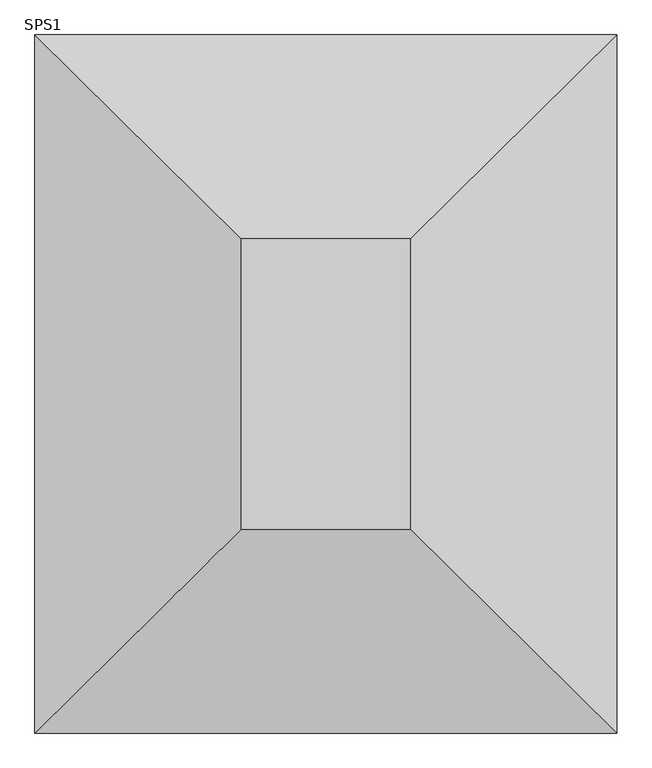
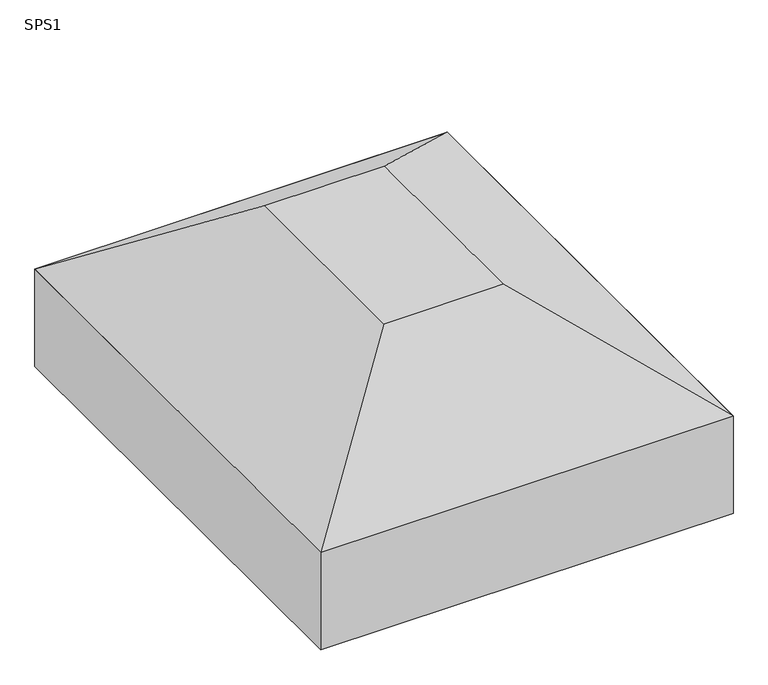
"""IFC4 building model written with IfcOpenShell, lengths in millimetres: fastener geometry, TQS - Sapata : SPS1."""

import ifcopenshell
import ifcopenshell.guid

model = None  # the IFC model being written
_history = None  # IfcOwnerHistory: only IFC2X3 demands one
_inside = {}  # id of a spatial element -> (the spatial element, [elements in it])
_under = {}  # id of a project, library or spatial element -> (it, [spatial elements below it])
_declared = {}  # id of a project -> (the project, [libraries it declares])
_typed = {}  # id of a type object -> (the type object, [elements of that type])
_made_of = {}  # id of a material, layer set ... -> (it, [elements and type objects made of it])


def new_model(schema):
    """Start an empty IFC model of exactly this schema.

    Asked for "IFC4X3", IfcOpenShell would pick the latest addendum, in which some entities
    have other attributes; the version numbers below select the first issue.
    IFC2X3 requires an IfcOwnerHistory on every rooted entity: one is made here for all.
    """
    global model, _history
    if schema == "IFC4X3":
        model = ifcopenshell.file(schema_version=(4, 3, 0, 0))
    else:
        model = ifcopenshell.file(schema=schema)
    _inside.clear()
    _under.clear()
    _declared.clear()
    _typed.clear()
    _made_of.clear()
    _history = None
    if model.schema == "IFC2X3":
        org = make("IfcOrganization", Name="unknown")
        user = make(
            "IfcPersonAndOrganization",
            ThePerson=make("IfcPerson", FamilyName="unknown"),
            TheOrganization=org,
        )
        app = make(
            "IfcApplication",
            ApplicationDeveloper=org,
            Version="unknown",
            ApplicationFullName="unknown",
            ApplicationIdentifier="unknown",
        )
        _history = make(
            "IfcOwnerHistory",
            OwningUser=user,
            OwningApplication=app,
            ChangeAction="ADDED",
            CreationDate=0,
        )
    return model


def make(cls, **values):
    """One entity of the class cls with the attributes given. An attribute that is None is left unset."""
    return model.create_entity(
        cls, **{name: value for name, value in values.items() if value is not None}
    )


def rooted(cls, **values):
    """An entity with a GlobalId (a new one), such as an element, a storey or a relation."""
    return make(cls, GlobalId=ifcopenshell.guid.new(), OwnerHistory=_history, **values)


def si_unit(unit_type, name, prefix=None):
    """IfcSIUnit, for example si_unit("LENGTHUNIT", "METRE", prefix="MILLI")."""
    return make("IfcSIUnit", UnitType=unit_type, Prefix=prefix, Name=name)


def assignment(units):
    """IfcUnitAssignment: the units of a project."""
    return None if units is None else make("IfcUnitAssignment", Units=units)


def point(xyz):
    """IfcCartesianPoint."""
    return None if xyz is None else make("IfcCartesianPoint", Coordinates=xyz)


def direction(xyz):
    """IfcDirection."""
    return None if xyz is None else make("IfcDirection", DirectionRatios=xyz)


def frame(location, z_axis=None, x_axis=None):
    """IfcAxis2Placement3D, a coordinate frame: its origin and axes. An axis left out is left unset."""
    return make(
        "IfcAxis2Placement3D",
        Location=point(location),
        Axis=direction(z_axis),
        RefDirection=direction(x_axis),
    )


def origin():
    """The frame at (0, 0, 0) with its axes left unset."""
    return frame((0.0, 0.0, 0.0))


def place(relative_to, where):
    """IfcLocalPlacement: puts the frame where relative to a parent placement (None: the world)."""
    return make(
        "IfcLocalPlacement", PlacementRelTo=relative_to, RelativePlacement=where
    )


def context(
    kind, dimensions, precision=None, world=None, true_north=None, identifier=None
):
    """IfcGeometricRepresentationContext, for example the 3D "Model" context."""
    return make(
        "IfcGeometricRepresentationContext",
        ContextIdentifier=identifier,
        ContextType=kind,
        CoordinateSpaceDimension=dimensions,
        Precision=precision,
        WorldCoordinateSystem=world,
        TrueNorth=true_north,
    )


def project(units=None, contexts=None):
    """IfcProject with its units and contexts."""
    return rooted(
        "IfcProject",
        Name="project",
        RepresentationContexts=contexts,
        UnitsInContext=assignment(units),
    )


def spatial(cls, under=None, at=None, **own):
    """A site, building, storey or space (cls), placed at a placement, below another one or the project."""
    s = rooted(cls, ObjectPlacement=at, **own)
    if under is not None:
        _under.setdefault(under.id(), (under, []))[1].append(s)
    return s


def polyline(points):
    """IfcPolyline through the points."""
    return make("IfcPolyline", Points=[point(p) for p in points])


def outline(outer, holes=None, kind="AREA"):
    """IfcArbitraryClosedProfileDef: a profile drawn as a closed curve; with holes, ...WithVoids."""
    if holes is None:
        return make("IfcArbitraryClosedProfileDef", ProfileType=kind, OuterCurve=outer)
    return make(
        "IfcArbitraryProfileDefWithVoids",
        ProfileType=kind,
        OuterCurve=outer,
        InnerCurves=holes,
    )


def extrude(swept, where, along, depth):
    """IfcExtrudedAreaSolid: the profile swept, set in the frame where, extruded along a direction by depth."""
    return make(
        "IfcExtrudedAreaSolid",
        SweptArea=swept,
        Position=where,
        ExtrudedDirection=direction(along),
        Depth=depth,
    )


def faces_of(points, faces, orient=None, outer=None):
    """IfcFace entities. A face is a list of loops; a loop is a list of indices into points, from 0.

    orient and outer hold one flag for each loop. By default every Orientation is true, the
    first loop of a face is its IfcFaceOuterBound and the others are IfcFaceBound.
    """
    made = []
    for i, loops in enumerate(faces):
        bounds = []
        for j, loop in enumerate(loops):
            is_outer = j == 0 if outer is None else outer[i][j]
            bounds.append(
                make(
                    "IfcFaceOuterBound" if is_outer else "IfcFaceBound",
                    Bound=make("IfcPolyLoop", Polygon=[points[k] for k in loop]),
                    Orientation=True if orient is None else orient[i][j],
                )
            )
        made.append(make("IfcFace", Bounds=bounds))
    return made


def faceted_brep(points, faces, orient=None, outer=None, voids=None):
    """IfcFacetedBrep: a solid bounded by flat faces; with voids (closed shells), ...WithVoids."""
    shared = [point(p) for p in points]
    hull = make("IfcClosedShell", CfsFaces=faces_of(shared, faces, orient, outer))
    if voids is None:
        return make("IfcFacetedBrep", Outer=hull)
    return make(
        "IfcFacetedBrepWithVoids",
        Outer=hull,
        Voids=[
            make(cls, CfsFaces=faces_of(shared, fs, o, b)) for cls, fs, o, b in voids
        ],
    )


def shape(context_of_items, identifier, shape_type, items):
    """IfcShapeRepresentation: the items that make up one representation, for example the "Body"."""
    return make(
        "IfcShapeRepresentation",
        ContextOfItems=context_of_items,
        RepresentationIdentifier=identifier,
        RepresentationType=shape_type,
        Items=items,
    )


def source(mapping_origin, context_of_items, identifier, shape_type, items):
    """IfcRepresentationMap: a shape defined once, which mapped items show again and again."""
    return make(
        "IfcRepresentationMap",
        MappingOrigin=mapping_origin,
        MappedRepresentation=shape(context_of_items, identifier, shape_type, items),
    )


def transform(
    local_origin,
    x_axis=None,
    y_axis=None,
    z_axis=None,
    scale=None,
    scale2=None,
    scale3=None,
    uniform=True,
):
    """IfcCartesianTransformationOperator3D, or its non-uniform kind. x_axis, y_axis, z_axis: its Axis1, 2, 3."""
    if uniform:
        return make(
            "IfcCartesianTransformationOperator3D",
            Axis1=direction(x_axis),
            Axis2=direction(y_axis),
            LocalOrigin=point(local_origin),
            Scale=scale,
            Axis3=direction(z_axis),
        )
    return make(
        "IfcCartesianTransformationOperator3DnonUniform",
        Axis1=direction(x_axis),
        Axis2=direction(y_axis),
        LocalOrigin=point(local_origin),
        Scale=scale,
        Axis3=direction(z_axis),
        Scale2=scale2,
        Scale3=scale3,
    )


def mapped(mapping_source, mapping_target):
    """IfcMappedItem: shows the shape of a source again, moved by a transform."""
    return make(
        "IfcMappedItem", MappingSource=mapping_source, MappingTarget=mapping_target
    )


def made_of(thing, what):
    """Note that an element or type object is made of a material, layer set ...; save() writes the relation."""
    if what is not None:
        _made_of.setdefault(what.id(), (what, []))[1].append(thing)
    return thing


def element(
    cls,
    number,
    at=None,
    inside=None,
    cuts=None,
    type_object=None,
    material=None,
    context=None,
    identifier="Body",
    shape_type=None,
    held_by="IfcProductDefinitionShape",
    body=None,
    shapes=None,
    **own,
):
    """One element of the class cls, such as IfcWall. Its Tag is "e" and its number.

    at: its placement. inside: the storey or other place that contains it. cuts: it is an
    opening in that element (IfcRelVoidsElement). A single representation is given by context,
    identifier, shape_type and body (its items); several are given by shapes. held_by: the class
    of the entity that holds the representations. save() writes the other relations.
    """
    e = rooted(cls, Tag="e%d" % number, ObjectPlacement=at, **own)
    if body is not None:
        shapes = [shape(context, identifier, shape_type, body)]
    if shapes is not None:
        e.Representation = make(held_by, Representations=shapes)
    if inside is not None:
        _inside.setdefault(inside.id(), (inside, []))[1].append(e)
    if cuts is not None:
        rooted(
            "IfcRelVoidsElement", RelatingBuildingElement=cuts, RelatedOpeningElement=e
        )
    if type_object is not None:
        _typed.setdefault(type_object.id(), (type_object, []))[1].append(e)
    return made_of(e, material)


def aggregate(whole, parts):
    """IfcRelAggregates: a whole, such as a stair, and the parts it consists of."""
    return rooted("IfcRelAggregates", RelatingObject=whole, RelatedObjects=parts)


def save(model, path):
    """Write the relations noted so far, then the file.

    IfcRelAggregates (storeys below a building ...), IfcRelContainedInSpatialStructure (elements
    in a storey), IfcRelDefinesByType, IfcRelAssociatesMaterial and IfcRelDeclares: one each for
    every whole, place, type object, material and project.
    """
    for whole, parts in _under.values():
        aggregate(whole, parts)
    for where, things in _inside.values():
        rooted(
            "IfcRelContainedInSpatialStructure",
            RelatedElements=things,
            RelatingStructure=where,
        )
    for kind, things in _typed.values():
        rooted("IfcRelDefinesByType", RelatedObjects=things, RelatingType=kind)
    for what, things in _made_of.values():
        rooted("IfcRelAssociatesMaterial", RelatedObjects=things, RelatingMaterial=what)
    for by, libraries in _declared.values():
        rooted("IfcRelDeclares", RelatingContext=by, RelatedDefinitions=libraries)
    model.write(path)


def sps1_6b3be553(model_context):
    return source(origin(), model_context, "Body", "SolidModel", [
        faceted_brep([(-55.0, 50.0, 0.0), (-345.0, 50.0, 0.0), (-345.0, -450.0, 0.0), (-55.0, -450.0, 0.0), (300.0, 400.0, -250.0), (300.0, -800.0, -250.0), (-700.0, -800.0, -250.0), (-700.0, 400.0, -250.0)], [[[0, 1, 2, 3]], [[4, 5, 6, 7]], [[4, 7, 1, 0]], [[7, 6, 2, 1]], [[6, 5, 3, 2]], [[5, 4, 0, 3]]]),
        extrude(outline(polyline([(300.0, 400.0), (300.0, -800.0), (-700.0, -800.0), (-700.0, 400.0), (300.0, 400.0)])), frame((0.0, 0.0, -500.0), z_axis=(0.0, 0.0, 1.0), x_axis=(1.0, 0.0, 0.0)), (0.0, 0.0, 1.0), 250.0),
    ])


if __name__ == "__main__":
    model = new_model("IFC4")
    model_context = context("Model", 3, world=origin())
    ifc_project = project(units=[si_unit("LENGTHUNIT", "METRE", prefix="MILLI")], contexts=[model_context])
    site = spatial("IfcSite", under=ifc_project)
    building = spatial("IfcBuilding", under=site)
    placement = place(None, origin())
    sps1_shape = sps1_6b3be553(model_context)
    element("IfcFastener", 1, ObjectType="TQS - Sapata : SPS1", at=placement, inside=building, context=model_context, shape_type="MappedRepresentation", body=[
        mapped(sps1_shape, transform((0.0, 0.0, 0.0), x_axis=(1.0, 0.0, 0.0), y_axis=(0.0, 1.0, 0.0), z_axis=(0.0, 0.0, 1.0))),
    ])
    save(model, "model.ifc")

# Revit data of these elements
# Type "TQS - Sapata : SPS1"
#   TY = 0.50 m
#   TX = 0.29 m
#   HS = 0.50 m
#   H0 = 0.25 m
#   EXCYABS = 0.60 m
#   EXCY = 0.00 m
#   EXCXABS = 0.50 m
#   EXCX = 0.00 m
#   DIMY = 1.20 m
#   DIMX = 1.00 m
#   Material estrutural = Concreto - Concreto concretado no local
#   Width = 0
#   Length = 0
# Element 1 (IfcFastener, "TQS - Sapata : SPS1")
#   Materials on its faces: "Concreto - Concreto concretado no local"
# Materials
#   "Concreto - Concreto concretado no local": class "Concreto", colour RGB 192 192 192, transparency 0
